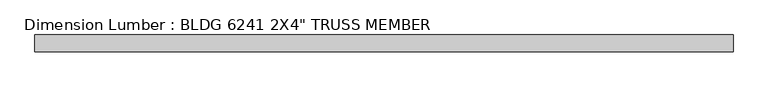
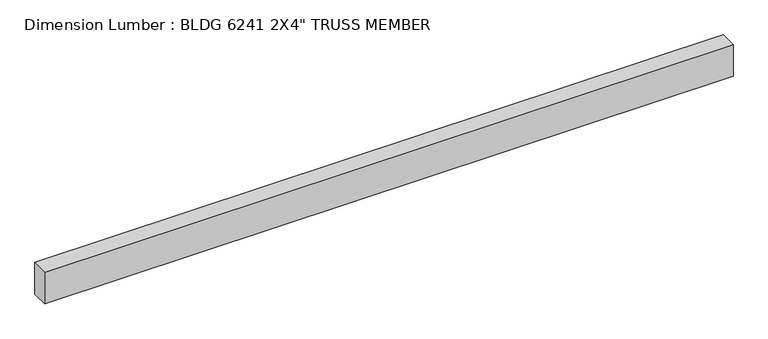
"""IFC4 building model written with IfcOpenShell, lengths in millimetres: beam geometry."""

from ifc_helpers import new_model, si_unit, frame, origin, place, context, project, spatial, polyline, outline, extrude, source, transform, mapped, element, save


def beam_0d910f0c(model_context):
    return source(origin(), model_context, "Body", "SweptSolid", [
        extrude(outline(polyline([(233.4866591, -25.4), (-1841.8619641, -25.4), (-1841.8619641, 25.4), (233.4866591, 25.4), (233.4866591, -25.4)])), frame((0.0, 0.0, -50.8), z_axis=(0.0, 0.0, 1.0), x_axis=(1.0, 0.0, 0.0)), (0.0, 0.0, 1.0), 101.6),
    ])


if __name__ == "__main__":
    model = new_model("IFC4")
    model_context = context("Model", 3, world=origin())
    ifc_project = project(units=[si_unit("LENGTHUNIT", "METRE", prefix="MILLI")], contexts=[model_context])
    site = spatial("IfcSite", under=ifc_project)
    building = spatial("IfcBuilding", under=site)
    placement = place(None, origin())
    beam_shape = beam_0d910f0c(model_context)
    element("IfcBeam", 1, ObjectType="Dimension Lumber : BLDG 6241 2X4\" TRUSS MEMBER", at=placement, inside=building, context=model_context, shape_type="MappedRepresentation", body=[
        mapped(beam_shape, transform((0.0, 0.0, 0.0), x_axis=(1.0, 0.0, 0.0), y_axis=(0.0, 1.0, 0.0), z_axis=(0.0, 0.0, 1.0))),
    ])
    save(model, "model.ifc")

# Revit data of these elements
# Type "Dimension Lumber : BLDG 6241 2X4\" TRUSS MEMBER"
#   Assembly Code = "B10"
#   A = 0.273472 SF
#   Length [instance default] = 5' - 0"
#   b = 0' - 2"
#   d = 0' - 4"
#   Structural Material [instance default] = Softwood, Lumber
# Element 1 (IfcBeam, "Dimension Lumber : BLDG 6241 2X4\" TRUSS MEMBER")
#   Materials on its faces: "Softwood, Lumber"
# Materials
#   "Softwood, Lumber": class "Wood", colour RGB 223 192 134, transparency 0, Description = "Pinus Echinata", Cost = 0
